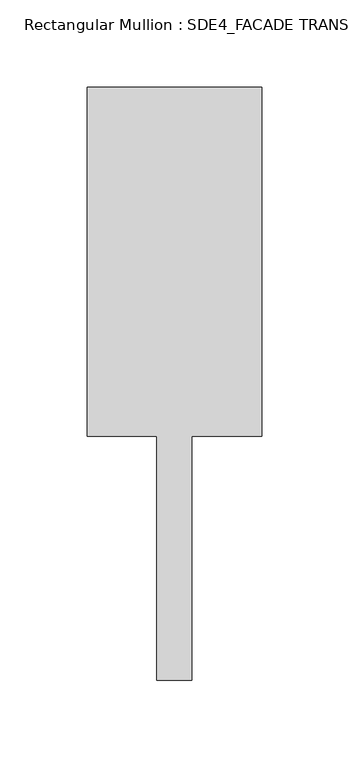
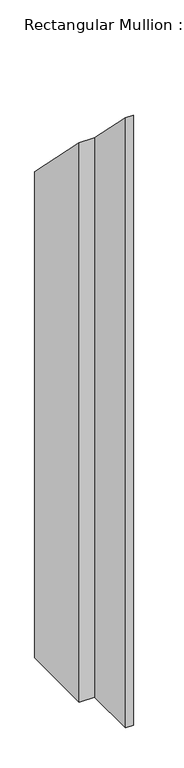
"""IFC4 building model written with IfcOpenShell, lengths in millimetres: member geometry, Rectangular Mullion : SDE4_FACADE TRANSOM TYPE 1."""

import ifcopenshell
import ifcopenshell.guid

model = None  # the IFC model being written
_history = None  # IfcOwnerHistory: only IFC2X3 demands one
_inside = {}  # id of a spatial element -> (the spatial element, [elements in it])
_under = {}  # id of a project, library or spatial element -> (it, [spatial elements below it])
_declared = {}  # id of a project -> (the project, [libraries it declares])
_typed = {}  # id of a type object -> (the type object, [elements of that type])
_made_of = {}  # id of a material, layer set ... -> (it, [elements and type objects made of it])


def new_model(schema):
    """Start an empty IFC model of exactly this schema.

    Asked for "IFC4X3", IfcOpenShell would pick the latest addendum, in which some entities
    have other attributes; the version numbers below select the first issue.
    IFC2X3 requires an IfcOwnerHistory on every rooted entity: one is made here for all.
    """
    global model, _history
    if schema == "IFC4X3":
        model = ifcopenshell.file(schema_version=(4, 3, 0, 0))
    else:
        model = ifcopenshell.file(schema=schema)
    _inside.clear()
    _under.clear()
    _declared.clear()
    _typed.clear()
    _made_of.clear()
    _history = None
    if model.schema == "IFC2X3":
        org = make("IfcOrganization", Name="unknown")
        user = make(
            "IfcPersonAndOrganization",
            ThePerson=make("IfcPerson", FamilyName="unknown"),
            TheOrganization=org,
        )
        app = make(
            "IfcApplication",
            ApplicationDeveloper=org,
            Version="unknown",
            ApplicationFullName="unknown",
            ApplicationIdentifier="unknown",
        )
        _history = make(
            "IfcOwnerHistory",
            OwningUser=user,
            OwningApplication=app,
            ChangeAction="ADDED",
            CreationDate=0,
        )
    return model


def make(cls, **values):
    """One entity of the class cls with the attributes given. An attribute that is None is left unset."""
    return model.create_entity(
        cls, **{name: value for name, value in values.items() if value is not None}
    )


def rooted(cls, **values):
    """An entity with a GlobalId (a new one), such as an element, a storey or a relation."""
    return make(cls, GlobalId=ifcopenshell.guid.new(), OwnerHistory=_history, **values)


def si_unit(unit_type, name, prefix=None):
    """IfcSIUnit, for example si_unit("LENGTHUNIT", "METRE", prefix="MILLI")."""
    return make("IfcSIUnit", UnitType=unit_type, Prefix=prefix, Name=name)


def assignment(units):
    """IfcUnitAssignment: the units of a project."""
    return None if units is None else make("IfcUnitAssignment", Units=units)


def point(xyz):
    """IfcCartesianPoint."""
    return None if xyz is None else make("IfcCartesianPoint", Coordinates=xyz)


def direction(xyz):
    """IfcDirection."""
    return None if xyz is None else make("IfcDirection", DirectionRatios=xyz)


def frame(location, z_axis=None, x_axis=None):
    """IfcAxis2Placement3D, a coordinate frame: its origin and axes. An axis left out is left unset."""
    return make(
        "IfcAxis2Placement3D",
        Location=point(location),
        Axis=direction(z_axis),
        RefDirection=direction(x_axis),
    )


def origin():
    """The frame at (0, 0, 0) with its axes left unset."""
    return frame((0.0, 0.0, 0.0))


def place(relative_to, where):
    """IfcLocalPlacement: puts the frame where relative to a parent placement (None: the world)."""
    return make(
        "IfcLocalPlacement", PlacementRelTo=relative_to, RelativePlacement=where
    )


def context(
    kind, dimensions, precision=None, world=None, true_north=None, identifier=None
):
    """IfcGeometricRepresentationContext, for example the 3D "Model" context."""
    return make(
        "IfcGeometricRepresentationContext",
        ContextIdentifier=identifier,
        ContextType=kind,
        CoordinateSpaceDimension=dimensions,
        Precision=precision,
        WorldCoordinateSystem=world,
        TrueNorth=true_north,
    )


def project(units=None, contexts=None):
    """IfcProject with its units and contexts."""
    return rooted(
        "IfcProject",
        Name="project",
        RepresentationContexts=contexts,
        UnitsInContext=assignment(units),
    )


def spatial(cls, under=None, at=None, **own):
    """A site, building, storey or space (cls), placed at a placement, below another one or the project."""
    s = rooted(cls, ObjectPlacement=at, **own)
    if under is not None:
        _under.setdefault(under.id(), (under, []))[1].append(s)
    return s


def faces_of(points, faces, orient=None, outer=None):
    """IfcFace entities. A face is a list of loops; a loop is a list of indices into points, from 0.

    orient and outer hold one flag for each loop. By default every Orientation is true, the
    first loop of a face is its IfcFaceOuterBound and the others are IfcFaceBound.
    """
    made = []
    for i, loops in enumerate(faces):
        bounds = []
        for j, loop in enumerate(loops):
            is_outer = j == 0 if outer is None else outer[i][j]
            bounds.append(
                make(
                    "IfcFaceOuterBound" if is_outer else "IfcFaceBound",
                    Bound=make("IfcPolyLoop", Polygon=[points[k] for k in loop]),
                    Orientation=True if orient is None else orient[i][j],
                )
            )
        made.append(make("IfcFace", Bounds=bounds))
    return made


def faceted_brep(points, faces, orient=None, outer=None, voids=None):
    """IfcFacetedBrep: a solid bounded by flat faces; with voids (closed shells), ...WithVoids."""
    shared = [point(p) for p in points]
    hull = make("IfcClosedShell", CfsFaces=faces_of(shared, faces, orient, outer))
    if voids is None:
        return make("IfcFacetedBrep", Outer=hull)
    return make(
        "IfcFacetedBrepWithVoids",
        Outer=hull,
        Voids=[
            make(cls, CfsFaces=faces_of(shared, fs, o, b)) for cls, fs, o, b in voids
        ],
    )


def shape(context_of_items, identifier, shape_type, items):
    """IfcShapeRepresentation: the items that make up one representation, for example the "Body"."""
    return make(
        "IfcShapeRepresentation",
        ContextOfItems=context_of_items,
        RepresentationIdentifier=identifier,
        RepresentationType=shape_type,
        Items=items,
    )


def source(mapping_origin, context_of_items, identifier, shape_type, items):
    """IfcRepresentationMap: a shape defined once, which mapped items show again and again."""
    return make(
        "IfcRepresentationMap",
        MappingOrigin=mapping_origin,
        MappedRepresentation=shape(context_of_items, identifier, shape_type, items),
    )


def transform(
    local_origin,
    x_axis=None,
    y_axis=None,
    z_axis=None,
    scale=None,
    scale2=None,
    scale3=None,
    uniform=True,
):
    """IfcCartesianTransformationOperator3D, or its non-uniform kind. x_axis, y_axis, z_axis: its Axis1, 2, 3."""
    if uniform:
        return make(
            "IfcCartesianTransformationOperator3D",
            Axis1=direction(x_axis),
            Axis2=direction(y_axis),
            LocalOrigin=point(local_origin),
            Scale=scale,
            Axis3=direction(z_axis),
        )
    return make(
        "IfcCartesianTransformationOperator3DnonUniform",
        Axis1=direction(x_axis),
        Axis2=direction(y_axis),
        LocalOrigin=point(local_origin),
        Scale=scale,
        Axis3=direction(z_axis),
        Scale2=scale2,
        Scale3=scale3,
    )


def mapped(mapping_source, mapping_target):
    """IfcMappedItem: shows the shape of a source again, moved by a transform."""
    return make(
        "IfcMappedItem", MappingSource=mapping_source, MappingTarget=mapping_target
    )


def made_of(thing, what):
    """Note that an element or type object is made of a material, layer set ...; save() writes the relation."""
    if what is not None:
        _made_of.setdefault(what.id(), (what, []))[1].append(thing)
    return thing


def element(
    cls,
    number,
    at=None,
    inside=None,
    cuts=None,
    type_object=None,
    material=None,
    context=None,
    identifier="Body",
    shape_type=None,
    held_by="IfcProductDefinitionShape",
    body=None,
    shapes=None,
    **own,
):
    """One element of the class cls, such as IfcWall. Its Tag is "e" and its number.

    at: its placement. inside: the storey or other place that contains it. cuts: it is an
    opening in that element (IfcRelVoidsElement). A single representation is given by context,
    identifier, shape_type and body (its items); several are given by shapes. held_by: the class
    of the entity that holds the representations. save() writes the other relations.
    """
    e = rooted(cls, Tag="e%d" % number, ObjectPlacement=at, **own)
    if body is not None:
        shapes = [shape(context, identifier, shape_type, body)]
    if shapes is not None:
        e.Representation = make(held_by, Representations=shapes)
    if inside is not None:
        _inside.setdefault(inside.id(), (inside, []))[1].append(e)
    if cuts is not None:
        rooted(
            "IfcRelVoidsElement", RelatingBuildingElement=cuts, RelatedOpeningElement=e
        )
    if type_object is not None:
        _typed.setdefault(type_object.id(), (type_object, []))[1].append(e)
    return made_of(e, material)


def aggregate(whole, parts):
    """IfcRelAggregates: a whole, such as a stair, and the parts it consists of."""
    return rooted("IfcRelAggregates", RelatingObject=whole, RelatedObjects=parts)


def save(model, path):
    """Write the relations noted so far, then the file.

    IfcRelAggregates (storeys below a building ...), IfcRelContainedInSpatialStructure (elements
    in a storey), IfcRelDefinesByType, IfcRelAssociatesMaterial and IfcRelDeclares: one each for
    every whole, place, type object, material and project.
    """
    for whole, parts in _under.values():
        aggregate(whole, parts)
    for where, things in _inside.values():
        rooted(
            "IfcRelContainedInSpatialStructure",
            RelatedElements=things,
            RelatingStructure=where,
        )
    for kind, things in _typed.values():
        rooted("IfcRelDefinesByType", RelatedObjects=things, RelatingType=kind)
    for what, things in _made_of.values():
        rooted("IfcRelAssociatesMaterial", RelatedObjects=things, RelatingMaterial=what)
    for by, libraries in _declared.values():
        rooted("IfcRelDeclares", RelatingContext=by, RelatedDefinitions=libraries)
    model.write(path)


def rectangular_mullion_sde4_facade_transom_type_1_2601b8c4(model_context):
    return source(origin(), model_context, "Body", "Brep", [
        faceted_brep([(50.0, 132.5, -1466.5), (50.0, -67.5, -1466.5), (10.0, -67.5, -1466.5), (10.0, -207.5, -1466.5), (-10.0, -207.5, -1466.5), (-10.0, -67.5, -1466.5), (-50.0, -67.5, -1466.5), (-50.0, 132.5, -1466.5), (-50.0, 132.5, -132.5), (50.0, 132.5, -132.5), (-50.0, -67.5, 67.5), (-10.0, -67.5, 67.5), (-10.0, -207.5, 207.5), (10.0, -207.5, 207.5), (10.0, -67.5, 67.5), (50.0, -67.5, 67.5)], [[[0, 1, 2, 3, 4, 5, 6, 7]], [[8, 9, 0, 7]], [[10, 8, 7, 6]], [[11, 10, 6, 5]], [[12, 11, 5, 4]], [[13, 12, 4, 3]], [[14, 13, 3, 2]], [[15, 14, 2, 1]], [[9, 15, 1, 0]], [[9, 8, 10, 11, 12, 13, 14, 15]]]),
    ])


if __name__ == "__main__":
    model = new_model("IFC4")
    model_context = context("Model", 3, world=origin())
    ifc_project = project(units=[si_unit("LENGTHUNIT", "METRE", prefix="MILLI")], contexts=[model_context])
    site = spatial("IfcSite", under=ifc_project)
    building = spatial("IfcBuilding", under=site)
    placement = place(None, origin())
    rectangular_mullion_sde4_facade_transom_type_1_shape = rectangular_mullion_sde4_facade_transom_type_1_2601b8c4(model_context)
    element("IfcMember", 1, ObjectType="Rectangular Mullion : SDE4_FACADE TRANSOM TYPE 1", at=placement, inside=building, context=model_context, shape_type="MappedRepresentation", body=[
        mapped(rectangular_mullion_sde4_facade_transom_type_1_shape, transform((0.0, 0.0, 0.0), x_axis=(1.0, 0.0, 0.0), y_axis=(0.0, 1.0, 0.0), z_axis=(0.0, 0.0, 1.0))),
    ])
    save(model, "model.ifc")

# Revit data of these elements
# Type "Rectangular Mullion : SDE4_FACADE TRANSOM TYPE 1"
#   built-in parameter 1007322 = 1.11549 (stored number, unit not read)
#   built-in parameter 1007321 = 0.164042 (stored number, unit not read)
#   built-in parameter 1007320 = 0.164042 (stored number, unit not read)
